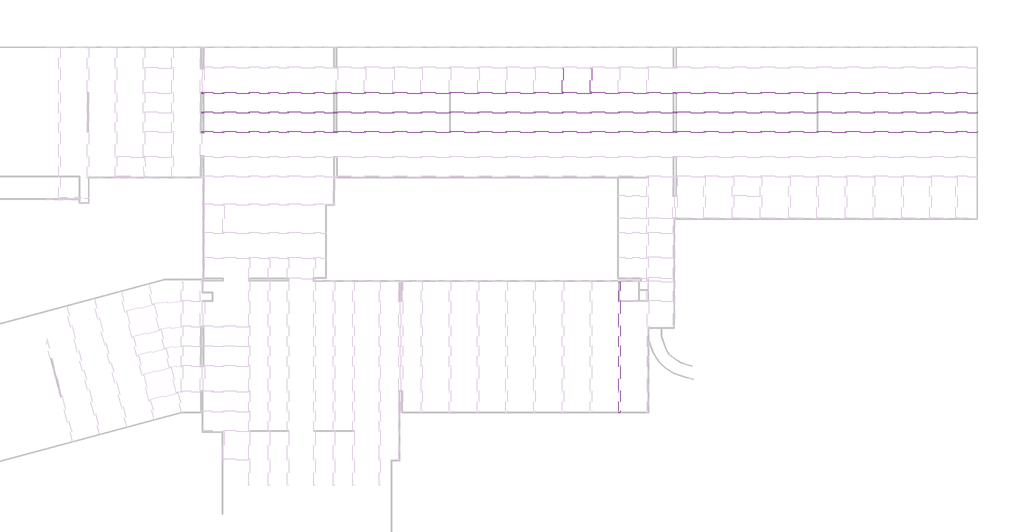
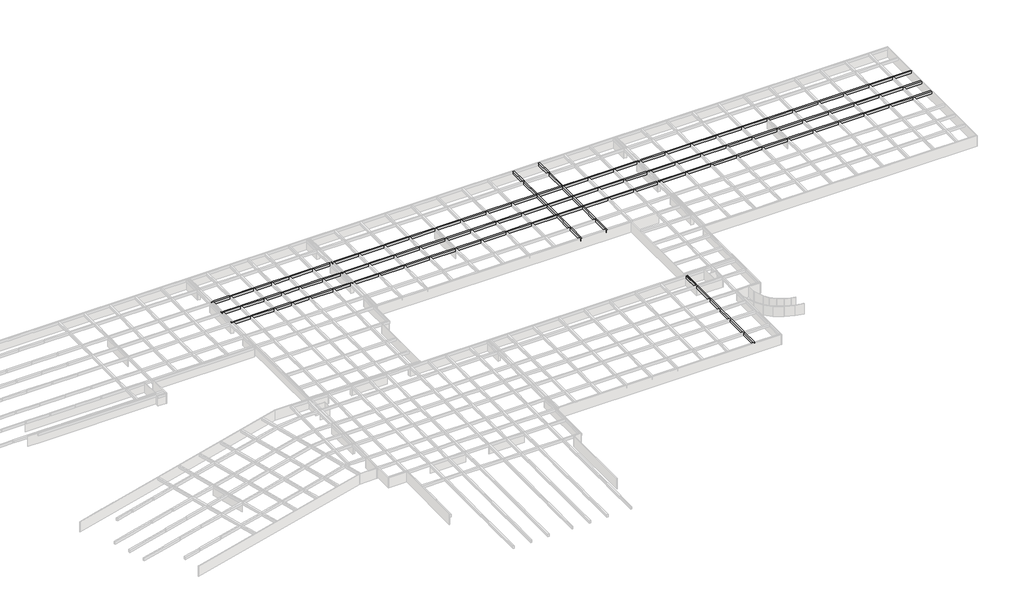
# One storey, part 12 of 14: 6 beams.
"""IFC4 building model written with IfcOpenShell, lengths in millimetres."""

from ifc_helpers import new_model, si_unit, frame, origin, place, context, project, spatial, polyline, outline, extrude, faceted_brep, element, save

model = new_model("IFC4")

# Units and contexts
model_context = context("Model", 3, world=origin())
ifc_project = project(units=[si_unit("LENGTHUNIT", "METRE", prefix="MILLI")], contexts=[model_context])

# Site, building, storey
site = spatial("IfcSite", under=ifc_project)
building = spatial("IfcBuilding", under=site)
storey = spatial("IfcBuildingStorey", under=building, Name="户型图", Elevation=0.0)

# Beams
placement = place(None, origin())
element("IfcBeam", 1, ObjectType="混凝土 - 矩形梁 : KL_beam", at=placement, inside=storey, context=model_context, shape_type="Brep", body=[
    faceted_brep([(227227.2949044, -129780.0179086, 3300.0), (227227.2949044, -130180.0179086, 3300.0), (227227.2949044, -130180.0179086, 2500.0), (227227.2949044, -129780.0179086, 2500.0), (221727.2949044, -129780.0179086, 3300.0), (221327.2949044, -129780.0179086, 3300.0), (214491.1566028, -129780.0179086, 3300.0), (214091.1566028, -129780.0179086, 3300.0), (206763.3308695, -129780.0179086, 3300.0), (206363.3308695, -129780.0179086, 3300.0), (198949.6658892, -129780.0179086, 3300.0), (198549.6658892, -129780.0179086, 3300.0), (191137.2949044, -129780.0179086, 3300.0), (190737.2949044, -129780.0179086, 3300.0), (183327.7006088, -129780.0179086, 3300.0), (182927.7006088, -129780.0179086, 3300.0), (175558.5232577, -129780.0179086, 3300.0), (175158.5232577, -129780.0179086, 3300.0), (167740.9658811, -129780.0179086, 3300.0), (167340.9658811, -129780.0179086, 3300.0), (159907.8874304, -129780.0179086, 3300.0), (159507.8874304, -129780.0179086, 3300.0), (152140.9658811, -129780.0179086, 3300.0), (151740.9658811, -129780.0179086, 3300.0), (144337.2949044, -129780.0179086, 3300.0), (143937.2949044, -129780.0179086, 3300.0), (143577.2949044, -129780.0179086, 3300.0), (143177.2949044, -129780.0179086, 3300.0), (136347.2949044, -129780.0179086, 3300.0), (135947.2949044, -129780.0179086, 3300.0), (128527.2949044, -129780.0179086, 3300.0), (128127.2949044, -129780.0179086, 3300.0), (120717.7893795, -129780.0179086, 3300.0), (120317.7893795, -129780.0179086, 3300.0), (112927.2949044, -129780.0179086, 3300.0), (112527.2949044, -129780.0179086, 3300.0), (105157.0968236, -129780.0179086, 3300.0), (104757.0968236, -129780.0179086, 3300.0), (97322.1026691, -129780.0179086, 3300.0), (96922.1026691, -129780.0179086, 3300.0), (89602.2949044, -129780.0179086, 3300.0), (89202.2949044, -129780.0179086, 3300.0), (81802.2949044, -129780.0179086, 3300.0), (81402.2949044, -129780.0179086, 3300.0), (73867.4871398, -129780.0179086, 3300.0), (73467.4871398, -129780.0179086, 3300.0), (66130.1134745, -129780.0179086, 3300.0), (65730.1134745, -129780.0179086, 3300.0), (58330.1134745, -129780.0179086, 3300.0), (57930.1134745, -129780.0179086, 3300.0), (50537.2949044, -129780.0179086, 3300.0), (50137.2949044, -129780.0179086, 3300.0), (49716.5330009, -129780.0179086, 3300.0), (49316.5330009, -129780.0179086, 3300.0), (44331.9066405, -129780.0179086, 3300.0), (43931.9066405, -129780.0179086, 3300.0), (37081.5607309, -129780.0179086, 3300.0), (36681.5607309, -129780.0179086, 3300.0), (31751.9066405, -129780.0179086, 3300.0), (31351.9066405, -129780.0179086, 3300.0), (26321.5607309, -129780.0179086, 3300.0), (25921.5607309, -129780.0179086, 3300.0), (19160.0865653, -129780.0179086, 3300.0), (18760.0865653, -129780.0179086, 3300.0), (13677.2949044, -129780.0179086, 3300.0), (13277.2949044, -129780.0179086, 3300.0), (12977.2949044, -129780.0179086, 3300.0), (12977.2949044, -130180.0179086, 3300.0), (13277.2949044, -130180.0179086, 3300.0), (13677.2949044, -130180.0179086, 3300.0), (18760.0865653, -130180.0179086, 3300.0), (19160.0865653, -130180.0179086, 3300.0), (25921.5607309, -130180.0179086, 3300.0), (26321.5607309, -130180.0179086, 3300.0), (31351.9066405, -130180.0179086, 3300.0), (31751.9066405, -130180.0179086, 3300.0), (36681.5607309, -130180.0179086, 3300.0), (37081.5607309, -130180.0179086, 3300.0), (43931.9066405, -130180.0179086, 3300.0), (44331.9066405, -130180.0179086, 3300.0), (49316.5330009, -130180.0179086, 3300.0), (49716.5330009, -130180.0179086, 3300.0), (50137.2949044, -130180.0179086, 3300.0), (50537.2949044, -130180.0179086, 3300.0), (57930.1134745, -130180.0179086, 3300.0), (58330.1134745, -130180.0179086, 3300.0), (65730.1134745, -130180.0179086, 3300.0), (66130.1134745, -130180.0179086, 3300.0), (73467.4871398, -130180.0179086, 3300.0), (73867.4871398, -130180.0179086, 3300.0), (81402.2949044, -130180.0179086, 3300.0), (81802.2949044, -130180.0179086, 3300.0), (89202.2949044, -130180.0179086, 3300.0), (89602.2949044, -130180.0179086, 3300.0), (96922.1026691, -130180.0179086, 3300.0), (97322.1026691, -130180.0179086, 3300.0), (104757.0968236, -130180.0179086, 3300.0), (105157.0968236, -130180.0179086, 3300.0), (112527.2949044, -130180.0179086, 3300.0), (112927.2949044, -130180.0179086, 3300.0), (120317.7893795, -130180.0179086, 3300.0), (120717.7893795, -130180.0179086, 3300.0), (128127.2949044, -130180.0179086, 3300.0), (128527.2949044, -130180.0179086, 3300.0), (135947.2949044, -130180.0179086, 3300.0), (136347.2949044, -130180.0179086, 3300.0), (143177.2949044, -130180.0179086, 3300.0), (143577.2949044, -130180.0179086, 3300.0), (143937.2949044, -130180.0179086, 3300.0), (144337.2949044, -130180.0179086, 3300.0), (151740.9658811, -130180.0179086, 3300.0), (152140.9658811, -130180.0179086, 3300.0), (159507.8874304, -130180.0179086, 3300.0), (159907.8874304, -130180.0179086, 3300.0), (167340.9658811, -130180.0179086, 3300.0), (167740.9658811, -130180.0179086, 3300.0), (175158.5232577, -130180.0179086, 3300.0), (175558.5232577, -130180.0179086, 3300.0), (182927.7006088, -130180.0179086, 3300.0), (183327.7006088, -130180.0179086, 3300.0), (190737.2949044, -130180.0179086, 3300.0), (191137.2949044, -130180.0179086, 3300.0), (198549.6658892, -130180.0179086, 3300.0), (198949.6658892, -130180.0179086, 3300.0), (206363.3308695, -130180.0179086, 3300.0), (206763.3308695, -130180.0179086, 3300.0), (214091.1566028, -130180.0179086, 3300.0), (214491.1566028, -130180.0179086, 3300.0), (221327.2949044, -130180.0179086, 3300.0), (221727.2949044, -130180.0179086, 3300.0), (12977.2949044, -130180.0179086, 2500.0), (13277.2949044, -130180.0179086, 2500.0), (13677.2949044, -130180.0179086, 2500.0), (18760.0865653, -130180.0179086, 2500.0), (19160.0865653, -130180.0179086, 2500.0), (25921.5607309, -130180.0179086, 2500.0), (26321.5607309, -130180.0179086, 2500.0), (31351.9066405, -130180.0179086, 2500.0), (31751.9066405, -130180.0179086, 2500.0), (36681.5607309, -130180.0179086, 2500.0), (37081.5607309, -130180.0179086, 2500.0), (43931.9066405, -130180.0179086, 2500.0), (44331.9066405, -130180.0179086, 2500.0), (49316.5330009, -130180.0179086, 2500.0), (49716.5330009, -130180.0179086, 2500.0), (50137.2949044, -130180.0179086, 2500.0), (50537.2949044, -130180.0179086, 2500.0), (57930.1134745, -130180.0179086, 2500.0), (58330.1134745, -130180.0179086, 2500.0), (65730.1134745, -130180.0179086, 2500.0), (66130.1134745, -130180.0179086, 2500.0), (73467.4871398, -130180.0179086, 2500.0), (73867.4871398, -130180.0179086, 2500.0), (81402.2949044, -130180.0179086, 2500.0), (81802.2949044, -130180.0179086, 2500.0), (89202.2949044, -130180.0179086, 2500.0), (89602.2949044, -130180.0179086, 2500.0), (96922.1026691, -130180.0179086, 2500.0), (97322.1026691, -130180.0179086, 2500.0), (104757.0968236, -130180.0179086, 2500.0), (105157.0968236, -130180.0179086, 2500.0), (112527.2949044, -130180.0179086, 2500.0), (112927.2949044, -130180.0179086, 2500.0), (120317.7893795, -130180.0179086, 2500.0), (120717.7893795, -130180.0179086, 2500.0), (128127.2949044, -130180.0179086, 2500.0), (128527.2949044, -130180.0179086, 2500.0), (135947.2949044, -130180.0179086, 2500.0), (136347.2949044, -130180.0179086, 2500.0), (143177.2949044, -130180.0179086, 2500.0), (143577.2949044, -130180.0179086, 2500.0), (143937.2949044, -130180.0179086, 2500.0), (144337.2949044, -130180.0179086, 2500.0), (151740.9658811, -130180.0179086, 2500.0), (152140.9658811, -130180.0179086, 2500.0), (159507.8874304, -130180.0179086, 2500.0), (159907.8874304, -130180.0179086, 2500.0), (167340.9658811, -130180.0179086, 2500.0), (167740.9658811, -130180.0179086, 2500.0), (175158.5232577, -130180.0179086, 2500.0), (175558.5232577, -130180.0179086, 2500.0), (182927.7006088, -130180.0179086, 2500.0), (183327.7006088, -130180.0179086, 2500.0), (190737.2949044, -130180.0179086, 2500.0), (191137.2949044, -130180.0179086, 2500.0), (198549.6658892, -130180.0179086, 2500.0), (198949.6658892, -130180.0179086, 2500.0), (206363.3308695, -130180.0179086, 2500.0), (206763.3308695, -130180.0179086, 2500.0), (214091.1566028, -130180.0179086, 2500.0), (214491.1566028, -130180.0179086, 2500.0), (221327.2949044, -130180.0179086, 2500.0), (221727.2949044, -130180.0179086, 2500.0), (12977.2949044, -129780.0179086, 2500.0), (13277.2949044, -129780.0179086, 2500.0), (13677.2949044, -129780.0179086, 2500.0), (18760.0865653, -129780.0179086, 2500.0), (19160.0865653, -129780.0179086, 2500.0), (25921.5607309, -129780.0179086, 2500.0), (26321.5607309, -129780.0179086, 2500.0), (31351.9066405, -129780.0179086, 2500.0), (31751.9066405, -129780.0179086, 2500.0), (36681.5607309, -129780.0179086, 2500.0), (37081.5607309, -129780.0179086, 2500.0), (43931.9066405, -129780.0179086, 2500.0), (44331.9066405, -129780.0179086, 2500.0), (49316.5330009, -129780.0179086, 2500.0), (49716.5330009, -129780.0179086, 2500.0), (50137.2949044, -129780.0179086, 2500.0), (50537.2949044, -129780.0179086, 2500.0), (57930.1134745, -129780.0179086, 2500.0), (58330.1134745, -129780.0179086, 2500.0), (65730.1134745, -129780.0179086, 2500.0), (66130.1134745, -129780.0179086, 2500.0), (73467.4871398, -129780.0179086, 2500.0), (73867.4871398, -129780.0179086, 2500.0), (81402.2949044, -129780.0179086, 2500.0), (81802.2949044, -129780.0179086, 2500.0), (89202.2949044, -129780.0179086, 2500.0), (89602.2949044, -129780.0179086, 2500.0), (96922.1026691, -129780.0179086, 2500.0), (97322.1026691, -129780.0179086, 2500.0), (104757.0968236, -129780.0179086, 2500.0), (105157.0968236, -129780.0179086, 2500.0), (112527.2949044, -129780.0179086, 2500.0), (112927.2949044, -129780.0179086, 2500.0), (120317.7893795, -129780.0179086, 2500.0), (120717.7893795, -129780.0179086, 2500.0), (128127.2949044, -129780.0179086, 2500.0), (128527.2949044, -129780.0179086, 2500.0), (135947.2949044, -129780.0179086, 2500.0), (136347.2949044, -129780.0179086, 2500.0), (143177.2949044, -129780.0179086, 2500.0), (143577.2949044, -129780.0179086, 2500.0), (143937.2949044, -129780.0179086, 2500.0), (144337.2949044, -129780.0179086, 2500.0), (151740.9658811, -129780.0179086, 2500.0), (152140.9658811, -129780.0179086, 2500.0), (159507.8874304, -129780.0179086, 2500.0), (159907.8874304, -129780.0179086, 2500.0), (167340.9658811, -129780.0179086, 2500.0), (167740.9658811, -129780.0179086, 2500.0), (175158.5232577, -129780.0179086, 2500.0), (175558.5232577, -129780.0179086, 2500.0), (182927.7006088, -129780.0179086, 2500.0), (183327.7006088, -129780.0179086, 2500.0), (190737.2949044, -129780.0179086, 2500.0), (191137.2949044, -129780.0179086, 2500.0), (198549.6658892, -129780.0179086, 2500.0), (198949.6658892, -129780.0179086, 2500.0), (206363.3308695, -129780.0179086, 2500.0), (206763.3308695, -129780.0179086, 2500.0), (214091.1566028, -129780.0179086, 2500.0), (214491.1566028, -129780.0179086, 2500.0), (221327.2949044, -129780.0179086, 2500.0), (221727.2949044, -129780.0179086, 2500.0)], [[[0, 1, 2, 3]], [[1, 0, 4, 5, 6, 7, 8, 9, 10, 11, 12, 13, 14, 15, 16, 17, 18, 19, 20, 21, 22, 23, 24, 25, 26, 27, 28, 29, 30, 31, 32, 33, 34, 35, 36, 37, 38, 39, 40, 41, 42, 43, 44, 45, 46, 47, 48, 49, 50, 51, 52, 53, 54, 55, 56, 57, 58, 59, 60, 61, 62, 63, 64, 65, 66, 67, 68, 69, 70, 71, 72, 73, 74, 75, 76, 77, 78, 79, 80, 81, 82, 83, 84, 85, 86, 87, 88, 89, 90, 91, 92, 93, 94, 95, 96, 97, 98, 99, 100, 101, 102, 103, 104, 105, 106, 107, 108, 109, 110, 111, 112, 113, 114, 115, 116, 117, 118, 119, 120, 121, 122, 123, 124, 125, 126, 127, 128, 129]], [[2, 1, 129, 128, 127, 126, 125, 124, 123, 122, 121, 120, 119, 118, 117, 116, 115, 114, 113, 112, 111, 110, 109, 108, 107, 106, 105, 104, 103, 102, 101, 100, 99, 98, 97, 96, 95, 94, 93, 92, 91, 90, 89, 88, 87, 86, 85, 84, 83, 82, 81, 80, 79, 78, 77, 76, 75, 74, 73, 72, 71, 70, 69, 68, 67, 130, 131, 132, 133, 134, 135, 136, 137, 138, 139, 140, 141, 142, 143, 144, 145, 146, 147, 148, 149, 150, 151, 152, 153, 154, 155, 156, 157, 158, 159, 160, 161, 162, 163, 164, 165, 166, 167, 168, 169, 170, 171, 172, 173, 174, 175, 176, 177, 178, 179, 180, 181, 182, 183, 184, 185, 186, 187, 188, 189, 190, 191, 192]], [[3, 2, 192, 191, 190, 189, 188, 187, 186, 185, 184, 183, 182, 181, 180, 179, 178, 177, 176, 175, 174, 173, 172, 171, 170, 169, 168, 167, 166, 165, 164, 163, 162, 161, 160, 159, 158, 157, 156, 155, 154, 153, 152, 151, 150, 149, 148, 147, 146, 145, 144, 143, 142, 141, 140, 139, 138, 137, 136, 135, 134, 133, 132, 131, 130, 193, 194, 195, 196, 197, 198, 199, 200, 201, 202, 203, 204, 205, 206, 207, 208, 209, 210, 211, 212, 213, 214, 215, 216, 217, 218, 219, 220, 221, 222, 223, 224, 225, 226, 227, 228, 229, 230, 231, 232, 233, 234, 235, 236, 237, 238, 239, 240, 241, 242, 243, 244, 245, 246, 247, 248, 249, 250, 251, 252, 253, 254, 255]], [[0, 3, 255, 254, 253, 252, 251, 250, 249, 248, 247, 246, 245, 244, 243, 242, 241, 240, 239, 238, 237, 236, 235, 234, 233, 232, 231, 230, 229, 228, 227, 226, 225, 224, 223, 222, 221, 220, 219, 218, 217, 216, 215, 214, 213, 212, 211, 210, 209, 208, 207, 206, 205, 204, 203, 202, 201, 200, 199, 198, 197, 196, 195, 194, 193, 66, 65, 64, 63, 62, 61, 60, 59, 58, 57, 56, 55, 54, 53, 52, 51, 50, 49, 48, 47, 46, 45, 44, 43, 42, 41, 40, 39, 38, 37, 36, 35, 34, 33, 32, 31, 30, 29, 28, 27, 26, 25, 24, 23, 22, 21, 20, 19, 18, 17, 16, 15, 14, 13, 12, 11, 10, 9, 8, 7, 6, 5, 4]], [[67, 66, 193, 130]]]),
])
element("IfcBeam", 2, ObjectType="混凝土 - 矩形梁 : KL_beam", at=placement, inside=storey, context=model_context, shape_type="Brep", body=[
    faceted_brep([(227227.2949044, -135580.0179086, 3300.0), (227227.2949044, -135580.0179086, 2500.0), (227227.2949044, -135180.0179086, 2500.0), (227227.2949044, -135180.0179086, 3300.0), (221727.2949044, -135180.0179086, 3300.0), (221327.2949044, -135180.0179086, 3300.0), (214491.1566028, -135180.0179086, 3300.0), (214091.1566028, -135180.0179086, 3300.0), (206763.3308695, -135180.0179086, 3300.0), (206363.3308695, -135180.0179086, 3300.0), (198949.6658892, -135180.0179086, 3300.0), (198549.6658892, -135180.0179086, 3300.0), (191137.2949044, -135180.0179086, 3300.0), (190737.2949044, -135180.0179086, 3300.0), (183327.7006088, -135180.0179086, 3300.0), (182927.7006088, -135180.0179086, 3300.0), (175558.5232577, -135180.0179086, 3300.0), (175158.5232577, -135180.0179086, 3300.0), (167740.9658811, -135180.0179086, 3300.0), (167340.9658811, -135180.0179086, 3300.0), (159907.8874304, -135180.0179086, 3300.0), (159507.8874304, -135180.0179086, 3300.0), (152140.9658811, -135180.0179086, 3300.0), (151740.9658811, -135180.0179086, 3300.0), (144337.2949044, -135180.0179086, 3300.0), (143937.2949044, -135180.0179086, 3300.0), (143577.2949044, -135180.0179086, 3300.0), (143177.2949044, -135180.0179086, 3300.0), (136347.2949044, -135180.0179086, 3300.0), (135947.2949044, -135180.0179086, 3300.0), (128527.2949044, -135180.0179086, 3300.0), (128127.2949044, -135180.0179086, 3300.0), (120717.7893795, -135180.0179086, 3300.0), (120317.7893795, -135180.0179086, 3300.0), (112927.2949044, -135180.0179086, 3300.0), (112527.2949044, -135180.0179086, 3300.0), (105157.0968236, -135180.0179086, 3300.0), (104757.0968236, -135180.0179086, 3300.0), (97322.1026691, -135180.0179086, 3300.0), (96922.1026691, -135180.0179086, 3300.0), (89602.2949044, -135180.0179086, 3300.0), (89202.2949044, -135180.0179086, 3300.0), (81802.2949044, -135180.0179086, 3300.0), (81402.2949044, -135180.0179086, 3300.0), (73867.4871398, -135180.0179086, 3300.0), (73467.4871398, -135180.0179086, 3300.0), (66130.1134745, -135180.0179086, 3300.0), (65730.1134745, -135180.0179086, 3300.0), (58330.1134745, -135180.0179086, 3300.0), (57930.1134745, -135180.0179086, 3300.0), (50537.2949044, -135180.0179086, 3300.0), (50137.2949044, -135180.0179086, 3300.0), (49716.5330009, -135180.0179086, 3300.0), (49316.5330009, -135180.0179086, 3300.0), (44331.9066405, -135180.0179086, 3300.0), (43931.9066405, -135180.0179086, 3300.0), (37081.5607309, -135180.0179086, 3300.0), (36681.5607309, -135180.0179086, 3300.0), (31751.9066405, -135180.0179086, 3300.0), (31351.9066405, -135180.0179086, 3300.0), (26321.5607309, -135180.0179086, 3300.0), (25921.5607309, -135180.0179086, 3300.0), (19160.0865653, -135180.0179086, 3300.0), (18760.0865653, -135180.0179086, 3300.0), (13677.2949044, -135180.0179086, 3300.0), (13277.2949044, -135180.0179086, 3300.0), (12977.2949044, -135180.0179086, 3300.0), (12977.2949044, -135580.0179086, 3300.0), (13277.2949044, -135580.0179086, 3300.0), (13677.2949044, -135580.0179086, 3300.0), (18760.0865653, -135580.0179086, 3300.0), (19160.0865653, -135580.0179086, 3300.0), (25921.5607309, -135580.0179086, 3300.0), (26321.5607309, -135580.0179086, 3300.0), (31351.9066405, -135580.0179086, 3300.0), (31751.9066405, -135580.0179086, 3300.0), (36681.5607309, -135580.0179086, 3300.0), (37081.5607309, -135580.0179086, 3300.0), (43931.9066405, -135580.0179086, 3300.0), (44331.9066405, -135580.0179086, 3300.0), (49316.5330009, -135580.0179086, 3300.0), (49716.5330009, -135580.0179086, 3300.0), (50137.2949044, -135580.0179086, 3300.0), (50537.2949044, -135580.0179086, 3300.0), (57930.1134745, -135580.0179086, 3300.0), (58330.1134745, -135580.0179086, 3300.0), (65730.1134745, -135580.0179086, 3300.0), (66130.1134745, -135580.0179086, 3300.0), (73467.4871398, -135580.0179086, 3300.0), (73867.4871398, -135580.0179086, 3300.0), (81402.2949044, -135580.0179086, 3300.0), (81802.2949044, -135580.0179086, 3300.0), (89202.2949044, -135580.0179086, 3300.0), (89602.2949044, -135580.0179086, 3300.0), (96922.1026691, -135580.0179086, 3300.0), (97322.1026691, -135580.0179086, 3300.0), (104757.0968236, -135580.0179086, 3300.0), (105157.0968236, -135580.0179086, 3300.0), (112527.2949044, -135580.0179086, 3300.0), (112927.2949044, -135580.0179086, 3300.0), (120317.7893795, -135580.0179086, 3300.0), (120717.7893795, -135580.0179086, 3300.0), (128127.2949044, -135580.0179086, 3300.0), (128527.2949044, -135580.0179086, 3300.0), (135947.2949044, -135580.0179086, 3300.0), (136347.2949044, -135580.0179086, 3300.0), (143177.2949044, -135580.0179086, 3300.0), (143577.2949044, -135580.0179086, 3300.0), (143937.2949044, -135580.0179086, 3300.0), (144337.2949044, -135580.0179086, 3300.0), (151740.9658811, -135580.0179086, 3300.0), (152140.9658811, -135580.0179086, 3300.0), (159507.8874304, -135580.0179086, 3300.0), (159907.8874304, -135580.0179086, 3300.0), (167340.9658811, -135580.0179086, 3300.0), (167740.9658811, -135580.0179086, 3300.0), (175158.5232577, -135580.0179086, 3300.0), (175558.5232577, -135580.0179086, 3300.0), (182927.7006088, -135580.0179086, 3300.0), (183327.7006088, -135580.0179086, 3300.0), (190737.2949044, -135580.0179086, 3300.0), (191137.2949044, -135580.0179086, 3300.0), (198549.6658892, -135580.0179086, 3300.0), (198949.6658892, -135580.0179086, 3300.0), (206363.3308695, -135580.0179086, 3300.0), (206763.3308695, -135580.0179086, 3300.0), (214091.1566028, -135580.0179086, 3300.0), (214491.1566028, -135580.0179086, 3300.0), (221327.2949044, -135580.0179086, 3300.0), (221727.2949044, -135580.0179086, 3300.0), (221727.2949044, -135180.0179086, 2500.0), (221327.2949044, -135180.0179086, 2500.0), (214491.1566028, -135180.0179086, 2500.0), (214091.1566028, -135180.0179086, 2500.0), (206763.3308695, -135180.0179086, 2500.0), (206363.3308695, -135180.0179086, 2500.0), (198949.6658892, -135180.0179086, 2500.0), (198549.6658892, -135180.0179086, 2500.0), (191137.2949044, -135180.0179086, 2500.0), (190737.2949044, -135180.0179086, 2500.0), (183327.7006088, -135180.0179086, 2500.0), (182927.7006088, -135180.0179086, 2500.0), (175558.5232577, -135180.0179086, 2500.0), (175158.5232577, -135180.0179086, 2500.0), (167740.9658811, -135180.0179086, 2500.0), (167340.9658811, -135180.0179086, 2500.0), (159907.8874304, -135180.0179086, 2500.0), (159507.8874304, -135180.0179086, 2500.0), (152140.9658811, -135180.0179086, 2500.0), (151740.9658811, -135180.0179086, 2500.0), (144337.2949044, -135180.0179086, 2500.0), (143937.2949044, -135180.0179086, 2500.0), (143577.2949044, -135180.0179086, 2500.0), (143177.2949044, -135180.0179086, 2500.0), (136347.2949044, -135180.0179086, 2500.0), (135947.2949044, -135180.0179086, 2500.0), (128527.2949044, -135180.0179086, 2500.0), (128127.2949044, -135180.0179086, 2500.0), (120717.7893795, -135180.0179086, 2500.0), (120317.7893795, -135180.0179086, 2500.0), (112927.2949044, -135180.0179086, 2500.0), (112527.2949044, -135180.0179086, 2500.0), (105157.0968236, -135180.0179086, 2500.0), (104757.0968236, -135180.0179086, 2500.0), (97322.1026691, -135180.0179086, 2500.0), (96922.1026691, -135180.0179086, 2500.0), (89602.2949044, -135180.0179086, 2500.0), (89202.2949044, -135180.0179086, 2500.0), (81802.2949044, -135180.0179086, 2500.0), (81402.2949044, -135180.0179086, 2500.0), (73867.4871398, -135180.0179086, 2500.0), (73467.4871398, -135180.0179086, 2500.0), (66130.1134745, -135180.0179086, 2500.0), (65730.1134745, -135180.0179086, 2500.0), (58330.1134745, -135180.0179086, 2500.0), (57930.1134745, -135180.0179086, 2500.0), (50537.2949044, -135180.0179086, 2500.0), (50137.2949044, -135180.0179086, 2500.0), (49716.5330009, -135180.0179086, 2500.0), (49316.5330009, -135180.0179086, 2500.0), (44331.9066405, -135180.0179086, 2500.0), (43931.9066405, -135180.0179086, 2500.0), (37081.5607309, -135180.0179086, 2500.0), (36681.5607309, -135180.0179086, 2500.0), (31751.9066405, -135180.0179086, 2500.0), (31351.9066405, -135180.0179086, 2500.0), (26321.5607309, -135180.0179086, 2500.0), (25921.5607309, -135180.0179086, 2500.0), (19160.0865653, -135180.0179086, 2500.0), (18760.0865653, -135180.0179086, 2500.0), (13677.2949044, -135180.0179086, 2500.0), (13277.2949044, -135180.0179086, 2500.0), (12977.2949044, -135180.0179086, 2500.0), (221727.2949044, -135580.0179086, 2500.0), (221327.2949044, -135580.0179086, 2500.0), (214491.1566028, -135580.0179086, 2500.0), (214091.1566028, -135580.0179086, 2500.0), (206763.3308695, -135580.0179086, 2500.0), (206363.3308695, -135580.0179086, 2500.0), (198949.6658892, -135580.0179086, 2500.0), (198549.6658892, -135580.0179086, 2500.0), (191137.2949044, -135580.0179086, 2500.0), (190737.2949044, -135580.0179086, 2500.0), (183327.7006088, -135580.0179086, 2500.0), (182927.7006088, -135580.0179086, 2500.0), (175558.5232577, -135580.0179086, 2500.0), (175158.5232577, -135580.0179086, 2500.0), (167740.9658811, -135580.0179086, 2500.0), (167340.9658811, -135580.0179086, 2500.0), (159907.8874304, -135580.0179086, 2500.0), (159507.8874304, -135580.0179086, 2500.0), (152140.9658811, -135580.0179086, 2500.0), (151740.9658811, -135580.0179086, 2500.0), (144337.2949044, -135580.0179086, 2500.0), (143937.2949044, -135580.0179086, 2500.0), (143577.2949044, -135580.0179086, 2500.0), (143177.2949044, -135580.0179086, 2500.0), (136347.2949044, -135580.0179086, 2500.0), (135947.2949044, -135580.0179086, 2500.0), (128527.2949044, -135580.0179086, 2500.0), (128127.2949044, -135580.0179086, 2500.0), (120717.7893795, -135580.0179086, 2500.0), (120317.7893795, -135580.0179086, 2500.0), (112927.2949044, -135580.0179086, 2500.0), (112527.2949044, -135580.0179086, 2500.0), (105157.0968236, -135580.0179086, 2500.0), (104757.0968236, -135580.0179086, 2500.0), (97322.1026691, -135580.0179086, 2500.0), (96922.1026691, -135580.0179086, 2500.0), (89602.2949044, -135580.0179086, 2500.0), (89202.2949044, -135580.0179086, 2500.0), (81802.2949044, -135580.0179086, 2500.0), (81402.2949044, -135580.0179086, 2500.0), (73867.4871398, -135580.0179086, 2500.0), (73467.4871398, -135580.0179086, 2500.0), (66130.1134745, -135580.0179086, 2500.0), (65730.1134745, -135580.0179086, 2500.0), (58330.1134745, -135580.0179086, 2500.0), (57930.1134745, -135580.0179086, 2500.0), (50537.2949044, -135580.0179086, 2500.0), (50137.2949044, -135580.0179086, 2500.0), (49716.5330009, -135580.0179086, 2500.0), (49316.5330009, -135580.0179086, 2500.0), (44331.9066405, -135580.0179086, 2500.0), (43931.9066405, -135580.0179086, 2500.0), (37081.5607309, -135580.0179086, 2500.0), (36681.5607309, -135580.0179086, 2500.0), (31751.9066405, -135580.0179086, 2500.0), (31351.9066405, -135580.0179086, 2500.0), (26321.5607309, -135580.0179086, 2500.0), (25921.5607309, -135580.0179086, 2500.0), (19160.0865653, -135580.0179086, 2500.0), (18760.0865653, -135580.0179086, 2500.0), (13677.2949044, -135580.0179086, 2500.0), (13277.2949044, -135580.0179086, 2500.0), (12977.2949044, -135580.0179086, 2500.0)], [[[0, 1, 2, 3]], [[0, 3, 4, 5, 6, 7, 8, 9, 10, 11, 12, 13, 14, 15, 16, 17, 18, 19, 20, 21, 22, 23, 24, 25, 26, 27, 28, 29, 30, 31, 32, 33, 34, 35, 36, 37, 38, 39, 40, 41, 42, 43, 44, 45, 46, 47, 48, 49, 50, 51, 52, 53, 54, 55, 56, 57, 58, 59, 60, 61, 62, 63, 64, 65, 66, 67, 68, 69, 70, 71, 72, 73, 74, 75, 76, 77, 78, 79, 80, 81, 82, 83, 84, 85, 86, 87, 88, 89, 90, 91, 92, 93, 94, 95, 96, 97, 98, 99, 100, 101, 102, 103, 104, 105, 106, 107, 108, 109, 110, 111, 112, 113, 114, 115, 116, 117, 118, 119, 120, 121, 122, 123, 124, 125, 126, 127, 128, 129]], [[3, 2, 130, 131, 132, 133, 134, 135, 136, 137, 138, 139, 140, 141, 142, 143, 144, 145, 146, 147, 148, 149, 150, 151, 152, 153, 154, 155, 156, 157, 158, 159, 160, 161, 162, 163, 164, 165, 166, 167, 168, 169, 170, 171, 172, 173, 174, 175, 176, 177, 178, 179, 180, 181, 182, 183, 184, 185, 186, 187, 188, 189, 190, 191, 192, 66, 65, 64, 63, 62, 61, 60, 59, 58, 57, 56, 55, 54, 53, 52, 51, 50, 49, 48, 47, 46, 45, 44, 43, 42, 41, 40, 39, 38, 37, 36, 35, 34, 33, 32, 31, 30, 29, 28, 27, 26, 25, 24, 23, 22, 21, 20, 19, 18, 17, 16, 15, 14, 13, 12, 11, 10, 9, 8, 7, 6, 5, 4]], [[2, 1, 193, 194, 195, 196, 197, 198, 199, 200, 201, 202, 203, 204, 205, 206, 207, 208, 209, 210, 211, 212, 213, 214, 215, 216, 217, 218, 219, 220, 221, 222, 223, 224, 225, 226, 227, 228, 229, 230, 231, 232, 233, 234, 235, 236, 237, 238, 239, 240, 241, 242, 243, 244, 245, 246, 247, 248, 249, 250, 251, 252, 253, 254, 255, 192, 191, 190, 189, 188, 187, 186, 185, 184, 183, 182, 181, 180, 179, 178, 177, 176, 175, 174, 173, 172, 171, 170, 169, 168, 167, 166, 165, 164, 163, 162, 161, 160, 159, 158, 157, 156, 155, 154, 153, 152, 151, 150, 149, 148, 147, 146, 145, 144, 143, 142, 141, 140, 139, 138, 137, 136, 135, 134, 133, 132, 131, 130]], [[1, 0, 129, 128, 127, 126, 125, 124, 123, 122, 121, 120, 119, 118, 117, 116, 115, 114, 113, 112, 111, 110, 109, 108, 107, 106, 105, 104, 103, 102, 101, 100, 99, 98, 97, 96, 95, 94, 93, 92, 91, 90, 89, 88, 87, 86, 85, 84, 83, 82, 81, 80, 79, 78, 77, 76, 75, 74, 73, 72, 71, 70, 69, 68, 67, 255, 254, 253, 252, 251, 250, 249, 248, 247, 246, 245, 244, 243, 242, 241, 240, 239, 238, 237, 236, 235, 234, 233, 232, 231, 230, 229, 228, 227, 226, 225, 224, 223, 222, 221, 220, 219, 218, 217, 216, 215, 214, 213, 212, 211, 210, 209, 208, 207, 206, 205, 204, 203, 202, 201, 200, 199, 198, 197, 196, 195, 194, 193]], [[67, 66, 192, 255]]]),
])
element("IfcBeam", 3, ObjectType="混凝土 - 矩形梁 : KL_beam", at=placement, inside=storey, context=model_context, shape_type="Brep", body=[
    faceted_brep([(227227.2949044, -140520.0179086, 3300.0), (227227.2949044, -140920.0179086, 3300.0), (227227.2949044, -140920.0179086, 2500.0), (227227.2949044, -140520.0179086, 2500.0), (221727.2949044, -140520.0179086, 3300.0), (221327.2949044, -140520.0179086, 3300.0), (214491.1566028, -140520.0179086, 3300.0), (214091.1566028, -140520.0179086, 3300.0), (206763.3308695, -140520.0179086, 3300.0), (206363.3308695, -140520.0179086, 3300.0), (198949.6658892, -140520.0179086, 3300.0), (198549.6658892, -140520.0179086, 3300.0), (191137.2949044, -140520.0179086, 3300.0), (190737.2949044, -140520.0179086, 3300.0), (183327.7006088, -140520.0179086, 3300.0), (182927.7006088, -140520.0179086, 3300.0), (175558.5232577, -140520.0179086, 3300.0), (175158.5232577, -140520.0179086, 3300.0), (167740.9658811, -140520.0179086, 3300.0), (167340.9658811, -140520.0179086, 3300.0), (159907.8874304, -140520.0179086, 3300.0), (159507.8874304, -140520.0179086, 3300.0), (152140.9658811, -140520.0179086, 3300.0), (151740.9658811, -140520.0179086, 3300.0), (144337.2949044, -140520.0179086, 3300.0), (143937.2949044, -140520.0179086, 3300.0), (143577.2949044, -140520.0179086, 3300.0), (143177.2949044, -140520.0179086, 3300.0), (136347.2949044, -140520.0179086, 3300.0), (135947.2949044, -140520.0179086, 3300.0), (128527.2949044, -140520.0179086, 3300.0), (128127.2949044, -140520.0179086, 3300.0), (120717.7893795, -140520.0179086, 3300.0), (120317.7893795, -140520.0179086, 3300.0), (112927.2949044, -140520.0179086, 3300.0), (112527.2949044, -140520.0179086, 3300.0), (105157.0968236, -140520.0179086, 3300.0), (104757.0968236, -140520.0179086, 3300.0), (97322.1026691, -140520.0179086, 3300.0), (96922.1026691, -140520.0179086, 3300.0), (89602.2949044, -140520.0179086, 3300.0), (89202.2949044, -140520.0179086, 3300.0), (81802.2949044, -140520.0179086, 3300.0), (81402.2949044, -140520.0179086, 3300.0), (73867.4871398, -140520.0179086, 3300.0), (73467.4871398, -140520.0179086, 3300.0), (66130.1134745, -140520.0179086, 3300.0), (65730.1134745, -140520.0179086, 3300.0), (58330.1134745, -140520.0179086, 3300.0), (57930.1134745, -140520.0179086, 3300.0), (50537.2949044, -140520.0179086, 3300.0), (50137.2949044, -140520.0179086, 3300.0), (49716.5330009, -140520.0179086, 3300.0), (49316.5330009, -140520.0179086, 3300.0), (44331.9066405, -140520.0179086, 3300.0), (43931.9066405, -140520.0179086, 3300.0), (37081.5607309, -140520.0179086, 3300.0), (36681.5607309, -140520.0179086, 3300.0), (31751.9066405, -140520.0179086, 3300.0), (31351.9066405, -140520.0179086, 3300.0), (26321.5607309, -140520.0179086, 3300.0), (25921.5607309, -140520.0179086, 3300.0), (19160.0865653, -140520.0179086, 3300.0), (18760.0865653, -140520.0179086, 3300.0), (13677.2949044, -140520.0179086, 3300.0), (13277.2949044, -140520.0179086, 3300.0), (12977.2949044, -140520.0179086, 3300.0), (12977.2949044, -140920.0179086, 3300.0), (13277.2949044, -140920.0179086, 3300.0), (13677.2949044, -140920.0179086, 3300.0), (18760.0865653, -140920.0179086, 3300.0), (19160.0865653, -140920.0179086, 3300.0), (25921.5607309, -140920.0179086, 3300.0), (26321.5607309, -140920.0179086, 3300.0), (31351.9066405, -140920.0179086, 3300.0), (31751.9066405, -140920.0179086, 3300.0), (36681.5607309, -140920.0179086, 3300.0), (37081.5607309, -140920.0179086, 3300.0), (43931.9066405, -140920.0179086, 3300.0), (44331.9066405, -140920.0179086, 3300.0), (49316.5330009, -140920.0179086, 3300.0), (49716.5330009, -140920.0179086, 3300.0), (50137.2949044, -140920.0179086, 3300.0), (50537.2949044, -140920.0179086, 3300.0), (57930.1134745, -140920.0179086, 3300.0), (58330.1134745, -140920.0179086, 3300.0), (65730.1134745, -140920.0179086, 3300.0), (66130.1134745, -140920.0179086, 3300.0), (73467.4871398, -140920.0179086, 3300.0), (73867.4871398, -140920.0179086, 3300.0), (81402.2949044, -140920.0179086, 3300.0), (81802.2949044, -140920.0179086, 3300.0), (89202.2949044, -140920.0179086, 3300.0), (89602.2949044, -140920.0179086, 3300.0), (96922.1026691, -140920.0179086, 3300.0), (97322.1026691, -140920.0179086, 3300.0), (104757.0968236, -140920.0179086, 3300.0), (105157.0968236, -140920.0179086, 3300.0), (112527.2949044, -140920.0179086, 3300.0), (112927.2949044, -140920.0179086, 3300.0), (120317.7893795, -140920.0179086, 3300.0), (120717.7893795, -140920.0179086, 3300.0), (128127.2949044, -140920.0179086, 3300.0), (128527.2949044, -140920.0179086, 3300.0), (135947.2949044, -140920.0179086, 3300.0), (136347.2949044, -140920.0179086, 3300.0), (143177.2949044, -140920.0179086, 3300.0), (143577.2949044, -140920.0179086, 3300.0), (143937.2949044, -140920.0179086, 3300.0), (144337.2949044, -140920.0179086, 3300.0), (151740.9658811, -140920.0179086, 3300.0), (152140.9658811, -140920.0179086, 3300.0), (159507.8874304, -140920.0179086, 3300.0), (159907.8874304, -140920.0179086, 3300.0), (167340.9658811, -140920.0179086, 3300.0), (167740.9658811, -140920.0179086, 3300.0), (175158.5232577, -140920.0179086, 3300.0), (175558.5232577, -140920.0179086, 3300.0), (182927.7006088, -140920.0179086, 3300.0), (183327.7006088, -140920.0179086, 3300.0), (190737.2949044, -140920.0179086, 3300.0), (191137.2949044, -140920.0179086, 3300.0), (198549.6658892, -140920.0179086, 3300.0), (198949.6658892, -140920.0179086, 3300.0), (206363.3308695, -140920.0179086, 3300.0), (206763.3308695, -140920.0179086, 3300.0), (214091.1566028, -140920.0179086, 3300.0), (214491.1566028, -140920.0179086, 3300.0), (221327.2949044, -140920.0179086, 3300.0), (221727.2949044, -140920.0179086, 3300.0), (12977.2949044, -140920.0179086, 2500.0), (13277.2949044, -140920.0179086, 2500.0), (13677.2949044, -140920.0179086, 2500.0), (18760.0865653, -140920.0179086, 2500.0), (19160.0865653, -140920.0179086, 2500.0), (25921.5607309, -140920.0179086, 2500.0), (26321.5607309, -140920.0179086, 2500.0), (31351.9066405, -140920.0179086, 2500.0), (31751.9066405, -140920.0179086, 2500.0), (36681.5607309, -140920.0179086, 2500.0), (37081.5607309, -140920.0179086, 2500.0), (43931.9066405, -140920.0179086, 2500.0), (44331.9066405, -140920.0179086, 2500.0), (49316.5330009, -140920.0179086, 2500.0), (49716.5330009, -140920.0179086, 2500.0), (50137.2949044, -140920.0179086, 2500.0), (50537.2949044, -140920.0179086, 2500.0), (57930.1134745, -140920.0179086, 2500.0), (58330.1134745, -140920.0179086, 2500.0), (65730.1134745, -140920.0179086, 2500.0), (66130.1134745, -140920.0179086, 2500.0), (73467.4871398, -140920.0179086, 2500.0), (73867.4871398, -140920.0179086, 2500.0), (81402.2949044, -140920.0179086, 2500.0), (81802.2949044, -140920.0179086, 2500.0), (89202.2949044, -140920.0179086, 2500.0), (89602.2949044, -140920.0179086, 2500.0), (96922.1026691, -140920.0179086, 2500.0), (97322.1026691, -140920.0179086, 2500.0), (104757.0968236, -140920.0179086, 2500.0), (105157.0968236, -140920.0179086, 2500.0), (112527.2949044, -140920.0179086, 2500.0), (112927.2949044, -140920.0179086, 2500.0), (120317.7893795, -140920.0179086, 2500.0), (120717.7893795, -140920.0179086, 2500.0), (128127.2949044, -140920.0179086, 2500.0), (128527.2949044, -140920.0179086, 2500.0), (135947.2949044, -140920.0179086, 2500.0), (136347.2949044, -140920.0179086, 2500.0), (143177.2949044, -140920.0179086, 2500.0), (143577.2949044, -140920.0179086, 2500.0), (143937.2949044, -140920.0179086, 2500.0), (144337.2949044, -140920.0179086, 2500.0), (151740.9658811, -140920.0179086, 2500.0), (152140.9658811, -140920.0179086, 2500.0), (159507.8874304, -140920.0179086, 2500.0), (159907.8874304, -140920.0179086, 2500.0), (167340.9658811, -140920.0179086, 2500.0), (167740.9658811, -140920.0179086, 2500.0), (175158.5232577, -140920.0179086, 2500.0), (175558.5232577, -140920.0179086, 2500.0), (182927.7006088, -140920.0179086, 2500.0), (183327.7006088, -140920.0179086, 2500.0), (190737.2949044, -140920.0179086, 2500.0), (191137.2949044, -140920.0179086, 2500.0), (198549.6658892, -140920.0179086, 2500.0), (198949.6658892, -140920.0179086, 2500.0), (206363.3308695, -140920.0179086, 2500.0), (206763.3308695, -140920.0179086, 2500.0), (214091.1566028, -140920.0179086, 2500.0), (214491.1566028, -140920.0179086, 2500.0), (221327.2949044, -140920.0179086, 2500.0), (221727.2949044, -140920.0179086, 2500.0), (12977.2949044, -140520.0179086, 2500.0), (13277.2949044, -140520.0179086, 2500.0), (13677.2949044, -140520.0179086, 2500.0), (18760.0865653, -140520.0179086, 2500.0), (19160.0865653, -140520.0179086, 2500.0), (25921.5607309, -140520.0179086, 2500.0), (26321.5607309, -140520.0179086, 2500.0), (31351.9066405, -140520.0179086, 2500.0), (31751.9066405, -140520.0179086, 2500.0), (36681.5607309, -140520.0179086, 2500.0), (37081.5607309, -140520.0179086, 2500.0), (43931.9066405, -140520.0179086, 2500.0), (44331.9066405, -140520.0179086, 2500.0), (49316.5330009, -140520.0179086, 2500.0), (49716.5330009, -140520.0179086, 2500.0), (50137.2949044, -140520.0179086, 2500.0), (50537.2949044, -140520.0179086, 2500.0), (57930.1134745, -140520.0179086, 2500.0), (58330.1134745, -140520.0179086, 2500.0), (65730.1134745, -140520.0179086, 2500.0), (66130.1134745, -140520.0179086, 2500.0), (73467.4871398, -140520.0179086, 2500.0), (73867.4871398, -140520.0179086, 2500.0), (81402.2949044, -140520.0179086, 2500.0), (81802.2949044, -140520.0179086, 2500.0), (89202.2949044, -140520.0179086, 2500.0), (89602.2949044, -140520.0179086, 2500.0), (96922.1026691, -140520.0179086, 2500.0), (97322.1026691, -140520.0179086, 2500.0), (104757.0968236, -140520.0179086, 2500.0), (105157.0968236, -140520.0179086, 2500.0), (112527.2949044, -140520.0179086, 2500.0), (112927.2949044, -140520.0179086, 2500.0), (120317.7893795, -140520.0179086, 2500.0), (120717.7893795, -140520.0179086, 2500.0), (128127.2949044, -140520.0179086, 2500.0), (128527.2949044, -140520.0179086, 2500.0), (135947.2949044, -140520.0179086, 2500.0), (136347.2949044, -140520.0179086, 2500.0), (143177.2949044, -140520.0179086, 2500.0), (143577.2949044, -140520.0179086, 2500.0), (143937.2949044, -140520.0179086, 2500.0), (144337.2949044, -140520.0179086, 2500.0), (151740.9658811, -140520.0179086, 2500.0), (152140.9658811, -140520.0179086, 2500.0), (159507.8874304, -140520.0179086, 2500.0), (159907.8874304, -140520.0179086, 2500.0), (167340.9658811, -140520.0179086, 2500.0), (167740.9658811, -140520.0179086, 2500.0), (175158.5232577, -140520.0179086, 2500.0), (175558.5232577, -140520.0179086, 2500.0), (182927.7006088, -140520.0179086, 2500.0), (183327.7006088, -140520.0179086, 2500.0), (190737.2949044, -140520.0179086, 2500.0), (191137.2949044, -140520.0179086, 2500.0), (198549.6658892, -140520.0179086, 2500.0), (198949.6658892, -140520.0179086, 2500.0), (206363.3308695, -140520.0179086, 2500.0), (206763.3308695, -140520.0179086, 2500.0), (214091.1566028, -140520.0179086, 2500.0), (214491.1566028, -140520.0179086, 2500.0), (221327.2949044, -140520.0179086, 2500.0), (221727.2949044, -140520.0179086, 2500.0)], [[[0, 1, 2, 3]], [[1, 0, 4, 5, 6, 7, 8, 9, 10, 11, 12, 13, 14, 15, 16, 17, 18, 19, 20, 21, 22, 23, 24, 25, 26, 27, 28, 29, 30, 31, 32, 33, 34, 35, 36, 37, 38, 39, 40, 41, 42, 43, 44, 45, 46, 47, 48, 49, 50, 51, 52, 53, 54, 55, 56, 57, 58, 59, 60, 61, 62, 63, 64, 65, 66, 67, 68, 69, 70, 71, 72, 73, 74, 75, 76, 77, 78, 79, 80, 81, 82, 83, 84, 85, 86, 87, 88, 89, 90, 91, 92, 93, 94, 95, 96, 97, 98, 99, 100, 101, 102, 103, 104, 105, 106, 107, 108, 109, 110, 111, 112, 113, 114, 115, 116, 117, 118, 119, 120, 121, 122, 123, 124, 125, 126, 127, 128, 129]], [[2, 1, 129, 128, 127, 126, 125, 124, 123, 122, 121, 120, 119, 118, 117, 116, 115, 114, 113, 112, 111, 110, 109, 108, 107, 106, 105, 104, 103, 102, 101, 100, 99, 98, 97, 96, 95, 94, 93, 92, 91, 90, 89, 88, 87, 86, 85, 84, 83, 82, 81, 80, 79, 78, 77, 76, 75, 74, 73, 72, 71, 70, 69, 68, 67, 130, 131, 132, 133, 134, 135, 136, 137, 138, 139, 140, 141, 142, 143, 144, 145, 146, 147, 148, 149, 150, 151, 152, 153, 154, 155, 156, 157, 158, 159, 160, 161, 162, 163, 164, 165, 166, 167, 168, 169, 170, 171, 172, 173, 174, 175, 176, 177, 178, 179, 180, 181, 182, 183, 184, 185, 186, 187, 188, 189, 190, 191, 192]], [[3, 2, 192, 191, 190, 189, 188, 187, 186, 185, 184, 183, 182, 181, 180, 179, 178, 177, 176, 175, 174, 173, 172, 171, 170, 169, 168, 167, 166, 165, 164, 163, 162, 161, 160, 159, 158, 157, 156, 155, 154, 153, 152, 151, 150, 149, 148, 147, 146, 145, 144, 143, 142, 141, 140, 139, 138, 137, 136, 135, 134, 133, 132, 131, 130, 193, 194, 195, 196, 197, 198, 199, 200, 201, 202, 203, 204, 205, 206, 207, 208, 209, 210, 211, 212, 213, 214, 215, 216, 217, 218, 219, 220, 221, 222, 223, 224, 225, 226, 227, 228, 229, 230, 231, 232, 233, 234, 235, 236, 237, 238, 239, 240, 241, 242, 243, 244, 245, 246, 247, 248, 249, 250, 251, 252, 253, 254, 255]], [[0, 3, 255, 254, 253, 252, 251, 250, 249, 248, 247, 246, 245, 244, 243, 242, 241, 240, 239, 238, 237, 236, 235, 234, 233, 232, 231, 230, 229, 228, 227, 226, 225, 224, 223, 222, 221, 220, 219, 218, 217, 216, 215, 214, 213, 212, 211, 210, 209, 208, 207, 206, 205, 204, 203, 202, 201, 200, 199, 198, 197, 196, 195, 194, 193, 66, 65, 64, 63, 62, 61, 60, 59, 58, 57, 56, 55, 54, 53, 52, 51, 50, 49, 48, 47, 46, 45, 44, 43, 42, 41, 40, 39, 38, 37, 36, 35, 34, 33, 32, 31, 30, 29, 28, 27, 26, 25, 24, 23, 22, 21, 20, 19, 18, 17, 16, 15, 14, 13, 12, 11, 10, 9, 8, 7, 6, 5, 4]], [[67, 66, 193, 130]]]),
])
element("IfcBeam", 4, ObjectType="混凝土 - 矩形梁 : KL_beam", at=placement, inside=storey, context=model_context, shape_type="SweptSolid", body=[
    extrude(outline(polyline([(112927.2949044, -153358.950757), (112527.2949044, -153358.950757), (112527.2949044, -153299.284307), (112927.2949044, -153299.284307), (112927.2949044, -153358.950757)])), frame((0.0, 0.0, 2500.0), z_axis=(0.0, 0.0, 1.0), x_axis=(1.0, 0.0, 0.0)), (0.0, 0.0, 1.0), 800.0),
    extrude(outline(polyline([(112927.2949044, -122797.8127788), (112527.2949044, -122797.8127788), (112527.2949044, -117558.950757), (112927.2949044, -117558.950757), (112927.2949044, -122797.8127788)])), frame((0.0, 0.0, 2500.0), z_axis=(0.0, 0.0, 1.0), x_axis=(1.0, 0.0, 0.0)), (0.0, 0.0, 1.0), 800.0),
    extrude(outline(polyline([(112527.2949044, -123197.8127788), (112927.2949044, -123197.8127788), (112927.2949044, -129780.0179086), (112527.2949044, -129780.0179086), (112527.2949044, -123197.8127788)])), frame((0.0, 0.0, 2500.0), z_axis=(0.0, 0.0, 1.0), x_axis=(1.0, 0.0, 0.0)), (0.0, 0.0, 1.0), 800.0),
    extrude(outline(polyline([(112527.2949044, -130180.0179086), (112927.2949044, -130180.0179086), (112927.2949044, -135180.0179086), (112527.2949044, -135180.0179086), (112527.2949044, -130180.0179086)])), frame((0.0, 0.0, 2500.0), z_axis=(0.0, 0.0, 1.0), x_axis=(1.0, 0.0, 0.0)), (0.0, 0.0, 1.0), 800.0),
    extrude(outline(polyline([(112527.2949044, -135580.0179086), (112927.2949044, -135580.0179086), (112927.2949044, -140520.0179086), (112527.2949044, -140520.0179086), (112527.2949044, -135580.0179086)])), frame((0.0, 0.0, 2500.0), z_axis=(0.0, 0.0, 1.0), x_axis=(1.0, 0.0, 0.0)), (0.0, 0.0, 1.0), 800.0),
    extrude(outline(polyline([(112527.2949044, -140920.0179086), (112927.2949044, -140920.0179086), (112927.2949044, -147499.284307), (112527.2949044, -147499.284307), (112527.2949044, -140920.0179086)])), frame((0.0, 0.0, 2500.0), z_axis=(0.0, 0.0, 1.0), x_axis=(1.0, 0.0, 0.0)), (0.0, 0.0, 1.0), 800.0),
    extrude(outline(polyline([(112527.2949044, -147899.284307), (112927.2949044, -147899.284307), (112927.2949044, -152899.284307), (112527.2949044, -152899.284307), (112527.2949044, -147899.284307)])), frame((0.0, 0.0, 2500.0), z_axis=(0.0, 0.0, 1.0), x_axis=(1.0, 0.0, 0.0)), (0.0, 0.0, 1.0), 800.0),
])
element("IfcBeam", 5, ObjectType="混凝土 - 矩形梁 : KL_beam", at=placement, inside=storey, context=model_context, shape_type="SweptSolid", body=[
    extrude(outline(polyline([(120717.7893795, -153358.950757), (120317.7893795, -153358.950757), (120317.7893795, -153299.284307), (120717.7893795, -153299.284307), (120717.7893795, -153358.950757)])), frame((0.0, 0.0, 2500.0), z_axis=(0.0, 0.0, 1.0), x_axis=(1.0, 0.0, 0.0)), (0.0, 0.0, 1.0), 800.0),
    extrude(outline(polyline([(120317.7893795, -123197.8127788), (120717.7893795, -123197.8127788), (120717.7893795, -129780.0179086), (120317.7893795, -129780.0179086), (120317.7893795, -123197.8127788)])), frame((0.0, 0.0, 2500.0), z_axis=(0.0, 0.0, 1.0), x_axis=(1.0, 0.0, 0.0)), (0.0, 0.0, 1.0), 800.0),
    extrude(outline(polyline([(120717.7893795, -122797.8127788), (120317.7893795, -122797.8127788), (120317.7893795, -117558.950757), (120717.7893795, -117558.950757), (120717.7893795, -122797.8127788)])), frame((0.0, 0.0, 2500.0), z_axis=(0.0, 0.0, 1.0), x_axis=(1.0, 0.0, 0.0)), (0.0, 0.0, 1.0), 800.0),
    extrude(outline(polyline([(120317.7893795, -130180.0179086), (120717.7893795, -130180.0179086), (120717.7893795, -135180.0179086), (120317.7893795, -135180.0179086), (120317.7893795, -130180.0179086)])), frame((0.0, 0.0, 2500.0), z_axis=(0.0, 0.0, 1.0), x_axis=(1.0, 0.0, 0.0)), (0.0, 0.0, 1.0), 800.0),
    extrude(outline(polyline([(120317.7893795, -135580.0179086), (120717.7893795, -135580.0179086), (120717.7893795, -140520.0179086), (120317.7893795, -140520.0179086), (120317.7893795, -135580.0179086)])), frame((0.0, 0.0, 2500.0), z_axis=(0.0, 0.0, 1.0), x_axis=(1.0, 0.0, 0.0)), (0.0, 0.0, 1.0), 800.0),
    extrude(outline(polyline([(120317.7893795, -140920.0179086), (120717.7893795, -140920.0179086), (120717.7893795, -147499.284307), (120317.7893795, -147499.284307), (120317.7893795, -140920.0179086)])), frame((0.0, 0.0, 2500.0), z_axis=(0.0, 0.0, 1.0), x_axis=(1.0, 0.0, 0.0)), (0.0, 0.0, 1.0), 800.0),
    extrude(outline(polyline([(120317.7893795, -147899.284307), (120717.7893795, -147899.284307), (120717.7893795, -152899.284307), (120317.7893795, -152899.284307), (120317.7893795, -147899.284307)])), frame((0.0, 0.0, 2500.0), z_axis=(0.0, 0.0, 1.0), x_axis=(1.0, 0.0, 0.0)), (0.0, 0.0, 1.0), 800.0),
])
element("IfcBeam", 6, ObjectType="混凝土 - 矩形梁 : KL_beam", at=placement, inside=storey, context=model_context, shape_type="Brep", body=[
    faceted_brep([(128149.172254, -218258.950757, 3300.0), (128149.172254, -218258.950757, 2500.0), (128549.172254, -218258.950757, 2500.0), (128549.172254, -218258.950757, 3300.0), (128549.172254, -218208.950757, 3300.0), (128549.172254, -217808.950757, 3300.0), (128549.172254, -212708.950757, 3300.0), (128549.172254, -212308.950757, 3300.0), (128549.172254, -205576.1028577, 3300.0), (128549.172254, -205176.1028577, 3300.0), (128549.172254, -200154.952508, 3300.0), (128549.172254, -199754.952508, 3300.0), (128549.172254, -194741.3993539, 3300.0), (128549.172254, -194341.3993539, 3300.0), (128549.172254, -187598.950757, 3300.0), (128549.172254, -187198.950757, 3300.0), (128549.172254, -182068.950757, 3300.0), (128149.172254, -182068.950757, 3300.0), (128149.172254, -187198.950757, 3300.0), (128149.172254, -187598.950757, 3300.0), (128149.172254, -194341.3993539, 3300.0), (128149.172254, -194741.3993539, 3300.0), (128149.172254, -199754.952508, 3300.0), (128149.172254, -200154.952508, 3300.0), (128149.172254, -205176.1028577, 3300.0), (128149.172254, -205576.1028577, 3300.0), (128149.172254, -212308.950757, 3300.0), (128149.172254, -212708.950757, 3300.0), (128149.172254, -217808.950757, 3300.0), (128149.172254, -218208.950757, 3300.0), (128549.172254, -218208.950757, 2500.0), (128549.172254, -217808.950757, 2500.0), (128549.172254, -212708.950757, 2500.0), (128549.172254, -212308.950757, 2500.0), (128549.172254, -205576.1028577, 2500.0), (128549.172254, -205176.1028577, 2500.0), (128549.172254, -200154.952508, 2500.0), (128549.172254, -199754.952508, 2500.0), (128549.172254, -194741.3993539, 2500.0), (128549.172254, -194341.3993539, 2500.0), (128549.172254, -187598.950757, 2500.0), (128549.172254, -187198.950757, 2500.0), (128549.172254, -182068.950757, 2500.0), (128149.172254, -218208.950757, 2500.0), (128149.172254, -217808.950757, 2500.0), (128149.172254, -212708.950757, 2500.0), (128149.172254, -212308.950757, 2500.0), (128149.172254, -205576.1028577, 2500.0), (128149.172254, -205176.1028577, 2500.0), (128149.172254, -200154.952508, 2500.0), (128149.172254, -199754.952508, 2500.0), (128149.172254, -194741.3993539, 2500.0), (128149.172254, -194341.3993539, 2500.0), (128149.172254, -187598.950757, 2500.0), (128149.172254, -187198.950757, 2500.0), (128149.172254, -182068.950757, 2500.0)], [[[0, 1, 2, 3]], [[0, 3, 4, 5, 6, 7, 8, 9, 10, 11, 12, 13, 14, 15, 16, 17, 18, 19, 20, 21, 22, 23, 24, 25, 26, 27, 28, 29]], [[3, 2, 30, 31, 32, 33, 34, 35, 36, 37, 38, 39, 40, 41, 42, 16, 15, 14, 13, 12, 11, 10, 9, 8, 7, 6, 5, 4]], [[2, 1, 43, 44, 45, 46, 47, 48, 49, 50, 51, 52, 53, 54, 55, 42, 41, 40, 39, 38, 37, 36, 35, 34, 33, 32, 31, 30]], [[1, 0, 29, 28, 27, 26, 25, 24, 23, 22, 21, 20, 19, 18, 17, 55, 54, 53, 52, 51, 50, 49, 48, 47, 46, 45, 44, 43]], [[17, 16, 42, 55]]]),
])

save(model, "model.ifc")

# Revit data of these elements
# Type "混凝土 - 矩形梁 : KL_beam"
#   Length [instance default] = 1524 mm
#   b = 400 mm
#   h = 800 mm
#   Structural Material [instance default] = 混凝土 - 现场浇注混凝土
#   Assembly Code = ""
# Elements 1, 2, 3, 4, 5, 6 (IfcBeam, "混凝土 - 矩形梁 : KL_beam")
#   Comments = ""
#   Structural Material = none
#   Phase Created = 新构造
# Materials
#   "混凝土 - 现场浇注混凝土": class "混凝土", colour RGB 192 192 192, transparency 0
